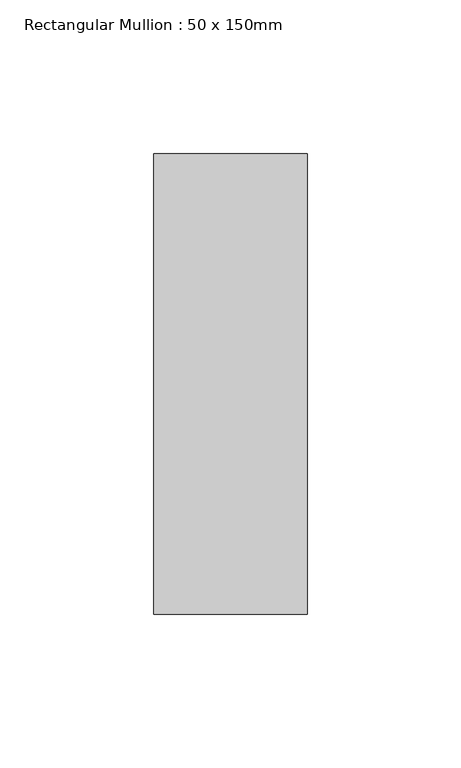
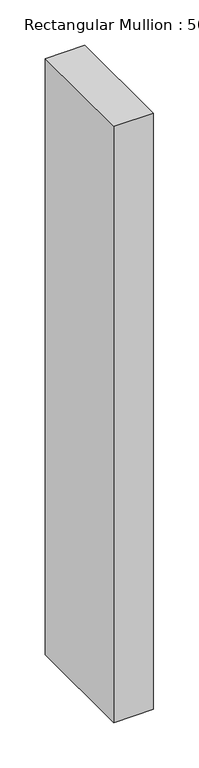
"""IFC4 building model written with IfcOpenShell, lengths in millimetres: member geometry, Rectangular Mullion : 50 x 150mm."""

from ifc_helpers import new_model, si_unit, frame, origin, place, context, project, spatial, polyline, outline, extrude, source, transform, mapped, element, save


def rectangular_mullion_50_x_150mm_14f10ac7(model_context):
    return source(origin(), model_context, "Body", "SweptSolid", [
        extrude(outline(polyline([(25.0, 75.0), (25.0, -75.0), (-25.0, -75.0), (-25.0, 75.0), (25.0, 75.0)])), frame((0.0, 0.0, -800.0), z_axis=(0.0, 0.0, 1.0), x_axis=(1.0, 0.0, 0.0)), (0.0, 0.0, 1.0), 800.0),
    ])


if __name__ == "__main__":
    model = new_model("IFC4")
    model_context = context("Model", 3, world=origin())
    ifc_project = project(units=[si_unit("LENGTHUNIT", "METRE", prefix="MILLI")], contexts=[model_context])
    site = spatial("IfcSite", under=ifc_project)
    building = spatial("IfcBuilding", under=site)
    placement = place(None, origin())
    rectangular_mullion_50_x_150mm_shape = rectangular_mullion_50_x_150mm_14f10ac7(model_context)
    element("IfcMember", 1, ObjectType="Rectangular Mullion : 50 x 150mm", at=placement, inside=building, context=model_context, shape_type="MappedRepresentation", body=[
        mapped(rectangular_mullion_50_x_150mm_shape, transform((0.0, 0.0, 0.0), x_axis=(1.0, 0.0, 0.0), y_axis=(0.0, 1.0, 0.0), z_axis=(0.0, 0.0, 1.0))),
    ])
    save(model, "model.ifc")

# Revit data of these elements
# Type "Rectangular Mullion : 50 x 150mm"
#   built-in parameter 1007304 = 0.492126 (stored number, unit not read)
#   built-in parameter 1007301 = 0.082021 (stored number, unit not read)
#   built-in parameter 1007300 = 0.082021 (stored number, unit not read)
# Element 1 (IfcMember, "Rectangular Mullion : 50 x 150mm")
#   Materials on its faces: "Metal - Aluminium"
# Materials
#   "Metal - Aluminium": class "Metal", colour RGB 247 247 247, transparency 0
